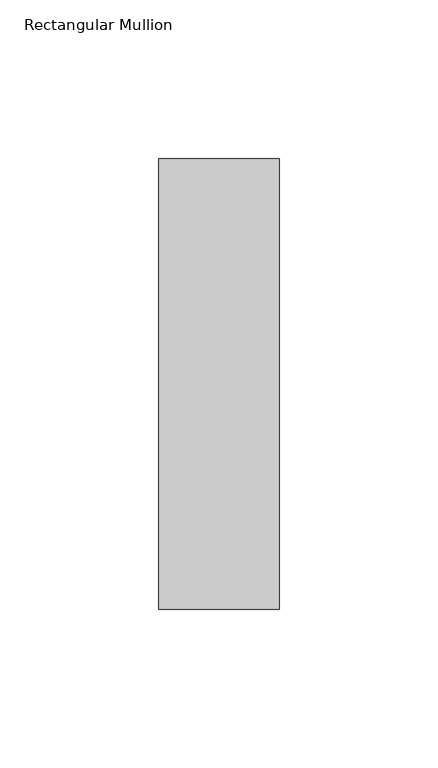
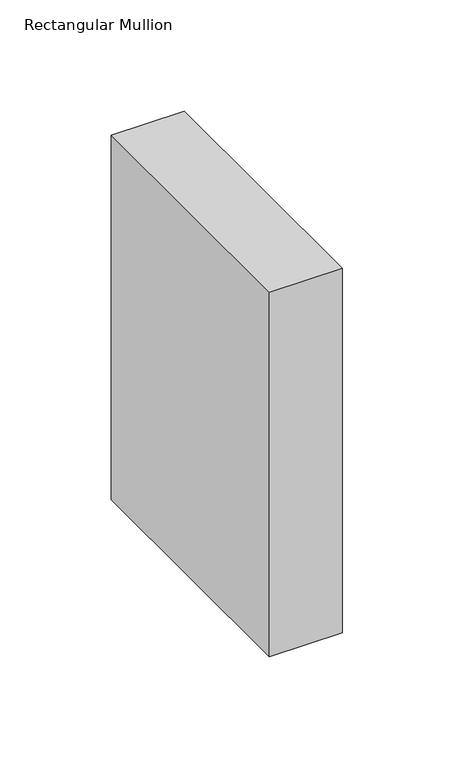
"""IFC4 building model written with IfcOpenShell, lengths in millimetres: member geometry, Rectangular Mullion : NLRS_21_CWM_hsb-regel 38x142_gen_rsf."""

import ifcopenshell
import ifcopenshell.guid

model = None  # the IFC model being written
_history = None  # IfcOwnerHistory: only IFC2X3 demands one
_inside = {}  # id of a spatial element -> (the spatial element, [elements in it])
_under = {}  # id of a project, library or spatial element -> (it, [spatial elements below it])
_declared = {}  # id of a project -> (the project, [libraries it declares])
_typed = {}  # id of a type object -> (the type object, [elements of that type])
_made_of = {}  # id of a material, layer set ... -> (it, [elements and type objects made of it])


def new_model(schema):
    """Start an empty IFC model of exactly this schema.

    Asked for "IFC4X3", IfcOpenShell would pick the latest addendum, in which some entities
    have other attributes; the version numbers below select the first issue.
    IFC2X3 requires an IfcOwnerHistory on every rooted entity: one is made here for all.
    """
    global model, _history
    if schema == "IFC4X3":
        model = ifcopenshell.file(schema_version=(4, 3, 0, 0))
    else:
        model = ifcopenshell.file(schema=schema)
    _inside.clear()
    _under.clear()
    _declared.clear()
    _typed.clear()
    _made_of.clear()
    _history = None
    if model.schema == "IFC2X3":
        org = make("IfcOrganization", Name="unknown")
        user = make(
            "IfcPersonAndOrganization",
            ThePerson=make("IfcPerson", FamilyName="unknown"),
            TheOrganization=org,
        )
        app = make(
            "IfcApplication",
            ApplicationDeveloper=org,
            Version="unknown",
            ApplicationFullName="unknown",
            ApplicationIdentifier="unknown",
        )
        _history = make(
            "IfcOwnerHistory",
            OwningUser=user,
            OwningApplication=app,
            ChangeAction="ADDED",
            CreationDate=0,
        )
    return model


def make(cls, **values):
    """One entity of the class cls with the attributes given. An attribute that is None is left unset."""
    return model.create_entity(
        cls, **{name: value for name, value in values.items() if value is not None}
    )


def rooted(cls, **values):
    """An entity with a GlobalId (a new one), such as an element, a storey or a relation."""
    return make(cls, GlobalId=ifcopenshell.guid.new(), OwnerHistory=_history, **values)


def si_unit(unit_type, name, prefix=None):
    """IfcSIUnit, for example si_unit("LENGTHUNIT", "METRE", prefix="MILLI")."""
    return make("IfcSIUnit", UnitType=unit_type, Prefix=prefix, Name=name)


def assignment(units):
    """IfcUnitAssignment: the units of a project."""
    return None if units is None else make("IfcUnitAssignment", Units=units)


def point(xyz):
    """IfcCartesianPoint."""
    return None if xyz is None else make("IfcCartesianPoint", Coordinates=xyz)


def direction(xyz):
    """IfcDirection."""
    return None if xyz is None else make("IfcDirection", DirectionRatios=xyz)


def frame(location, z_axis=None, x_axis=None):
    """IfcAxis2Placement3D, a coordinate frame: its origin and axes. An axis left out is left unset."""
    return make(
        "IfcAxis2Placement3D",
        Location=point(location),
        Axis=direction(z_axis),
        RefDirection=direction(x_axis),
    )


def origin():
    """The frame at (0, 0, 0) with its axes left unset."""
    return frame((0.0, 0.0, 0.0))


def place(relative_to, where):
    """IfcLocalPlacement: puts the frame where relative to a parent placement (None: the world)."""
    return make(
        "IfcLocalPlacement", PlacementRelTo=relative_to, RelativePlacement=where
    )


def context(
    kind, dimensions, precision=None, world=None, true_north=None, identifier=None
):
    """IfcGeometricRepresentationContext, for example the 3D "Model" context."""
    return make(
        "IfcGeometricRepresentationContext",
        ContextIdentifier=identifier,
        ContextType=kind,
        CoordinateSpaceDimension=dimensions,
        Precision=precision,
        WorldCoordinateSystem=world,
        TrueNorth=true_north,
    )


def project(units=None, contexts=None):
    """IfcProject with its units and contexts."""
    return rooted(
        "IfcProject",
        Name="project",
        RepresentationContexts=contexts,
        UnitsInContext=assignment(units),
    )


def spatial(cls, under=None, at=None, **own):
    """A site, building, storey or space (cls), placed at a placement, below another one or the project."""
    s = rooted(cls, ObjectPlacement=at, **own)
    if under is not None:
        _under.setdefault(under.id(), (under, []))[1].append(s)
    return s


def polyline(points):
    """IfcPolyline through the points."""
    return make("IfcPolyline", Points=[point(p) for p in points])


def outline(outer, holes=None, kind="AREA"):
    """IfcArbitraryClosedProfileDef: a profile drawn as a closed curve; with holes, ...WithVoids."""
    if holes is None:
        return make("IfcArbitraryClosedProfileDef", ProfileType=kind, OuterCurve=outer)
    return make(
        "IfcArbitraryProfileDefWithVoids",
        ProfileType=kind,
        OuterCurve=outer,
        InnerCurves=holes,
    )


def extrude(swept, where, along, depth):
    """IfcExtrudedAreaSolid: the profile swept, set in the frame where, extruded along a direction by depth."""
    return make(
        "IfcExtrudedAreaSolid",
        SweptArea=swept,
        Position=where,
        ExtrudedDirection=direction(along),
        Depth=depth,
    )


def shape(context_of_items, identifier, shape_type, items):
    """IfcShapeRepresentation: the items that make up one representation, for example the "Body"."""
    return make(
        "IfcShapeRepresentation",
        ContextOfItems=context_of_items,
        RepresentationIdentifier=identifier,
        RepresentationType=shape_type,
        Items=items,
    )


def source(mapping_origin, context_of_items, identifier, shape_type, items):
    """IfcRepresentationMap: a shape defined once, which mapped items show again and again."""
    return make(
        "IfcRepresentationMap",
        MappingOrigin=mapping_origin,
        MappedRepresentation=shape(context_of_items, identifier, shape_type, items),
    )


def transform(
    local_origin,
    x_axis=None,
    y_axis=None,
    z_axis=None,
    scale=None,
    scale2=None,
    scale3=None,
    uniform=True,
):
    """IfcCartesianTransformationOperator3D, or its non-uniform kind. x_axis, y_axis, z_axis: its Axis1, 2, 3."""
    if uniform:
        return make(
            "IfcCartesianTransformationOperator3D",
            Axis1=direction(x_axis),
            Axis2=direction(y_axis),
            LocalOrigin=point(local_origin),
            Scale=scale,
            Axis3=direction(z_axis),
        )
    return make(
        "IfcCartesianTransformationOperator3DnonUniform",
        Axis1=direction(x_axis),
        Axis2=direction(y_axis),
        LocalOrigin=point(local_origin),
        Scale=scale,
        Axis3=direction(z_axis),
        Scale2=scale2,
        Scale3=scale3,
    )


def mapped(mapping_source, mapping_target):
    """IfcMappedItem: shows the shape of a source again, moved by a transform."""
    return make(
        "IfcMappedItem", MappingSource=mapping_source, MappingTarget=mapping_target
    )


def made_of(thing, what):
    """Note that an element or type object is made of a material, layer set ...; save() writes the relation."""
    if what is not None:
        _made_of.setdefault(what.id(), (what, []))[1].append(thing)
    return thing


def element(
    cls,
    number,
    at=None,
    inside=None,
    cuts=None,
    type_object=None,
    material=None,
    context=None,
    identifier="Body",
    shape_type=None,
    held_by="IfcProductDefinitionShape",
    body=None,
    shapes=None,
    **own,
):
    """One element of the class cls, such as IfcWall. Its Tag is "e" and its number.

    at: its placement. inside: the storey or other place that contains it. cuts: it is an
    opening in that element (IfcRelVoidsElement). A single representation is given by context,
    identifier, shape_type and body (its items); several are given by shapes. held_by: the class
    of the entity that holds the representations. save() writes the other relations.
    """
    e = rooted(cls, Tag="e%d" % number, ObjectPlacement=at, **own)
    if body is not None:
        shapes = [shape(context, identifier, shape_type, body)]
    if shapes is not None:
        e.Representation = make(held_by, Representations=shapes)
    if inside is not None:
        _inside.setdefault(inside.id(), (inside, []))[1].append(e)
    if cuts is not None:
        rooted(
            "IfcRelVoidsElement", RelatingBuildingElement=cuts, RelatedOpeningElement=e
        )
    if type_object is not None:
        _typed.setdefault(type_object.id(), (type_object, []))[1].append(e)
    return made_of(e, material)


def aggregate(whole, parts):
    """IfcRelAggregates: a whole, such as a stair, and the parts it consists of."""
    return rooted("IfcRelAggregates", RelatingObject=whole, RelatedObjects=parts)


def save(model, path):
    """Write the relations noted so far, then the file.

    IfcRelAggregates (storeys below a building ...), IfcRelContainedInSpatialStructure (elements
    in a storey), IfcRelDefinesByType, IfcRelAssociatesMaterial and IfcRelDeclares: one each for
    every whole, place, type object, material and project.
    """
    for whole, parts in _under.values():
        aggregate(whole, parts)
    for where, things in _inside.values():
        rooted(
            "IfcRelContainedInSpatialStructure",
            RelatedElements=things,
            RelatingStructure=where,
        )
    for kind, things in _typed.values():
        rooted("IfcRelDefinesByType", RelatedObjects=things, RelatingType=kind)
    for what, things in _made_of.values():
        rooted("IfcRelAssociatesMaterial", RelatedObjects=things, RelatingMaterial=what)
    for by, libraries in _declared.values():
        rooted("IfcRelDeclares", RelatingContext=by, RelatedDefinitions=libraries)
    model.write(path)


def rectangular_mullion_cea15bcf(model_context):
    return source(origin(), model_context, "Body", "SweptSolid", [
        extrude(outline(polyline([(-38.0, -71.0), (-38.0, 71.0), (0.0, 71.0), (0.0, -71.0), (-38.0, -71.0)])), frame((0.0, 0.0, -199.9999997), z_axis=(0.0, 0.0, 1.0), x_axis=(1.0, 0.0, 0.0)), (0.0, 0.0, 1.0), 199.9999997),
    ])


if __name__ == "__main__":
    model = new_model("IFC4")
    model_context = context("Model", 3, world=origin())
    ifc_project = project(units=[si_unit("LENGTHUNIT", "METRE", prefix="MILLI")], contexts=[model_context])
    site = spatial("IfcSite", under=ifc_project)
    building = spatial("IfcBuilding", under=site)
    placement = place(None, origin())
    rectangular_mullion_shape = rectangular_mullion_cea15bcf(model_context)
    element("IfcMember", 1, ObjectType="Rectangular Mullion : NLRS_21_CWM_hsb-regel 38x142_gen_rsf", at=placement, inside=building, context=model_context, shape_type="MappedRepresentation", body=[
        mapped(rectangular_mullion_shape, transform((0.0, 0.0, 0.0), x_axis=(1.0, 0.0, 0.0), y_axis=(0.0, 1.0, 0.0), z_axis=(0.0, 0.0, 1.0))),
    ])
    save(model, "model.ifc")

# Revit data of these elements
# Type "Rectangular Mullion : NLRS_21_CWM_hsb-regel 38x142_gen_rsf"
#   Export Type to IFC As = "IfcWall"
#   Type IfcGUID = "07M7mRoiH1CR8m_RSKIwpF"
#   Assembly Code = "21.10"
#   built-in parameter 1007322 = 0.465879 (stored number, unit not read)
#   built-in parameter 1007321 = 0.062336 (stored number, unit not read)
#   built-in parameter 1007320 = 0.062336 (stored number, unit not read)
# Element 1 (IfcMember, "Rectangular Mullion : NLRS_21_CWM_hsb-regel 38x142_gen_rsf")
#   Materials on its faces: "NLRS_i2_hout naaldhout vuren_gen_rsf"
# Materials
#   "NLRS_i2_hout naaldhout vuren_gen_rsf": class "I - Hout", colour RGB 234 199 147, transparency 0, Keynote = "i2", Manufacturer = "Revit Standards Foundation", URL = "www.revitstandards.org", Description = "hout vuren", Cost = 0
